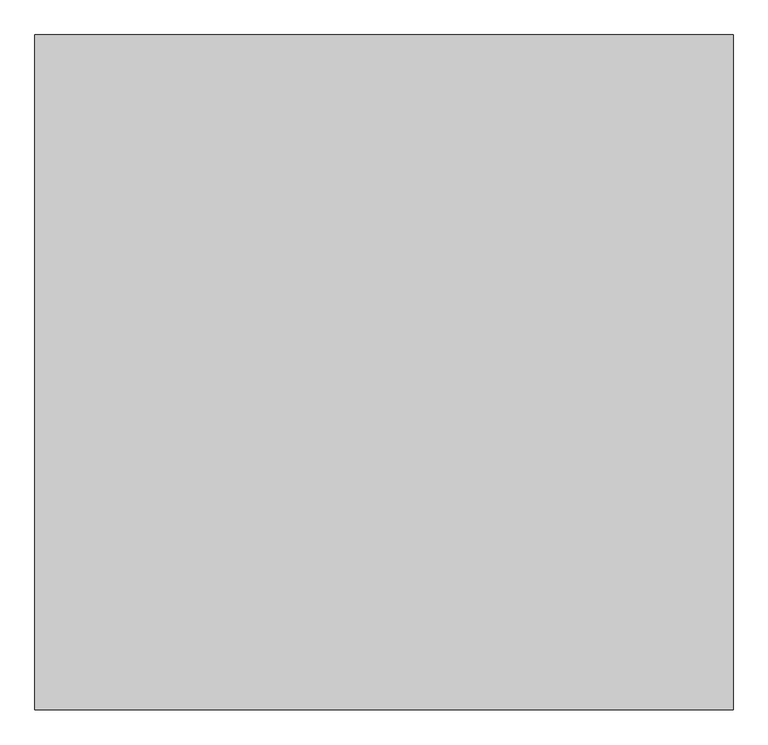
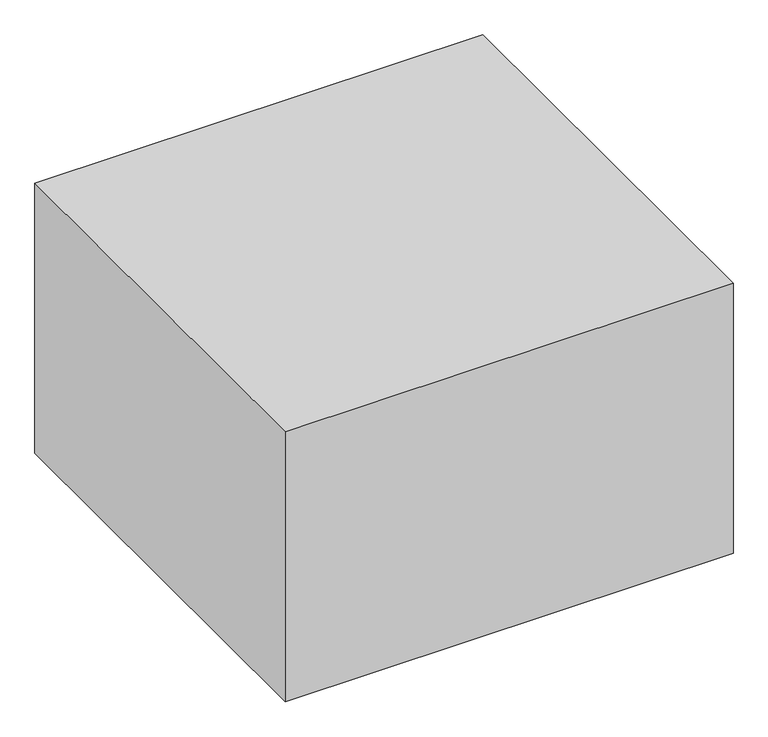
"""IFC4 building model written with IfcOpenShell, lengths in millimetres: proxy geometry, 0_3d."""

from ifc_helpers import new_model, si_unit, origin, origin_with_axes, place, context, project, spatial, polyline, outline, extrude, source, transform, mapped, element, save


def generic_models_5c66ab55(model_context):
    return source(origin(), model_context, "Body", "SweptSolid", [
        extrude(outline(polyline([(0.0, 0.0), (0.0, 4370.0), (4520.0, 4370.0), (4520.0, 0.0), (0.0, 0.0)])), origin_with_axes(), (0.0, 0.0, 1.0), 2880.0),
    ])


if __name__ == "__main__":
    model = new_model("IFC4")
    model_context = context("Model", 3, world=origin())
    ifc_project = project(units=[si_unit("LENGTHUNIT", "METRE", prefix="MILLI")], contexts=[model_context])
    site = spatial("IfcSite", under=ifc_project)
    building = spatial("IfcBuilding", under=site)
    placement = place(None, origin())
    generic_models_shape = generic_models_5c66ab55(model_context)
    element("IfcBuildingElementProxy", 1, Name="0_3d", ObjectType="0_3d", at=placement, inside=building, context=model_context, shape_type="MappedRepresentation", body=[
        mapped(generic_models_shape, transform((0.0, 0.0, 0.0), x_axis=(1.0, 0.0, 0.0), y_axis=(0.0, 1.0, 0.0), z_axis=(0.0, 0.0, 1.0))),
    ])
    save(model, "model.ifc")

# Revit data of these elements
# Element 1 (IfcBuildingElementProxy, "0_3d")
#   Materials on its faces: "*1"
# Materials
#   "*1": class "Unassigned", colour RGB 175 175 175, transparency 0
